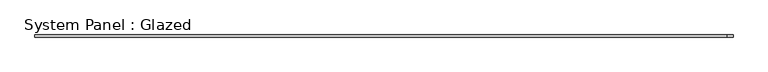
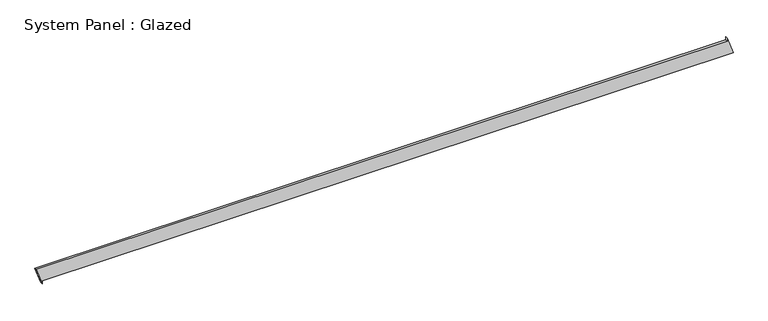
"""IFC4 building model written with IfcOpenShell, lengths in millimetres: plate geometry, System Panel : Glazed."""

from ifc_helpers import new_model, si_unit, frame, origin, place, context, project, spatial, polyline, outline, extrude, source, transform, mapped, element, save


def system_panel_glazed_6fd4334b(model_context):
    return source(origin(), model_context, "Body", "SweptSolid", [
        extrude(outline(polyline([(0.0, -3956.9205184), (35.3553391, -3956.9205184), (35.3553391, 4027.0701191), (235.2094887, 3957.0820623), (199.8541496, 3957.0823635), (199.7861186, -4027.0701191), (0.0, -3956.9205184)])), frame((0.0, -49.5, 0.0), z_axis=(0.0, 1.0, 0.0), x_axis=(0.0, 0.0, 1.0)), (0.0, 0.0, 1.0), 25.0),
    ])


if __name__ == "__main__":
    model = new_model("IFC4")
    model_context = context("Model", 3, world=origin())
    ifc_project = project(units=[si_unit("LENGTHUNIT", "METRE", prefix="MILLI")], contexts=[model_context])
    site = spatial("IfcSite", under=ifc_project)
    building = spatial("IfcBuilding", under=site)
    placement = place(None, origin())
    system_panel_glazed_shape = system_panel_glazed_6fd4334b(model_context)
    element("IfcPlate", 1, ObjectType="System Panel : Glazed", at=placement, inside=building, context=model_context, shape_type="MappedRepresentation", body=[
        mapped(system_panel_glazed_shape, transform((0.0, 0.0, 0.0), x_axis=(1.0, 0.0, 0.0), y_axis=(0.0, 1.0, 0.0), z_axis=(0.0, 0.0, 1.0))),
    ])
    save(model, "model.ifc")

# Revit data of these elements
# Element 1 (IfcPlate, "System Panel : Glazed")
#   Materials on its faces: "Glass"
# Materials
#   "Glass": class "Glass", colour RGB 218 227 224, transparency 0.85, Description = "Soda Lime Glass", Cost = 0
